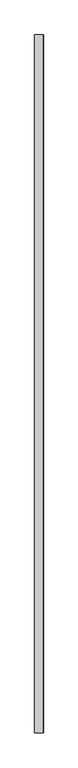
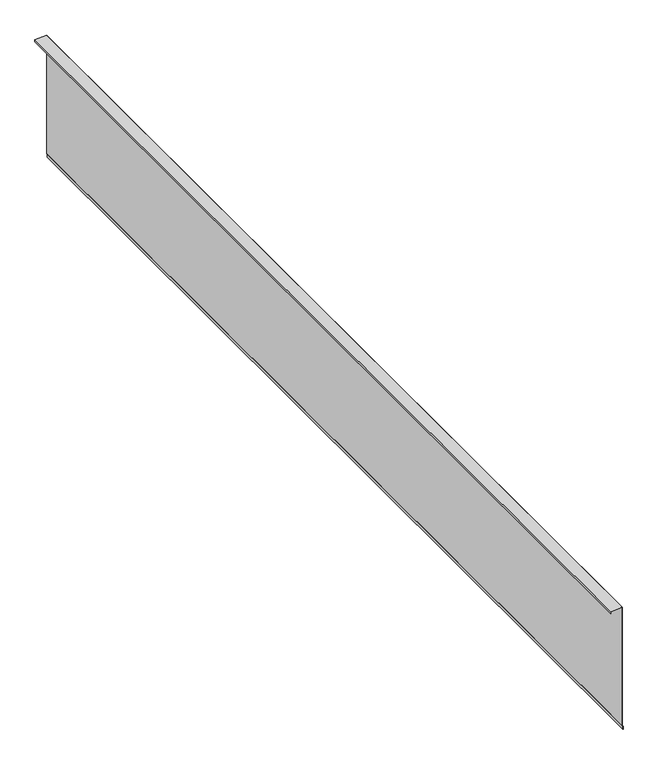
"""IFC4 building model written with IfcOpenShell, lengths in millimetres: proxy geometry, Generic Models 7:Generic Models 1:5:Generic Models 1:5 : Generic Models 7:Generic Models 1:337419:28 : Generic Models 7:Generic Models 1:5:Generic Models 1:5 : Generic Models 7:Generic Models 1:337419:311462."""

from ifc_helpers import new_model, si_unit, frame, origin, place, context, project, spatial, polyline, outline, extrude, source, transform, mapped, element, save


def generic_models_722ccff6(model_context):
    return source(origin(), model_context, "Body", "SweptSolid", [
        extrude(outline(polyline([(0.0, 0.0), (20.1758441, -1e-07), (64.4371907, 30.9921285), (65.3477433, 29.6917246), (20.6763809, -1.5875), (0.5005368, -1.5875), (-1952.5403074, -1369.1214216), (-2070.4890131, -1180.3640352), (-2034.5717889, -1155.2145241), (-2033.6612363, -1156.514928), (-2068.3444233, -1180.8003569), (-1952.0805203, -1366.8614955), (0.0, 0.0)])), frame((579321.2054739, -579019.7413841, 3795.8885169), z_axis=(1.0439982212062661e-11, 1.0, 0.0), x_axis=(0.5735764363524188, -5.988127792777543e-12, -0.8191520442880308)), (0.0, 0.0, 1.0), 18974.5924408),
    ])


if __name__ == "__main__":
    model = new_model("IFC4")
    model_context = context("Model", 3, world=origin())
    ifc_project = project(units=[si_unit("LENGTHUNIT", "METRE", prefix="MILLI")], contexts=[model_context])
    site = spatial("IfcSite", under=ifc_project)
    building = spatial("IfcBuilding", under=site)
    placement = place(None, origin())
    generic_models_shape = generic_models_722ccff6(model_context)
    element("IfcBuildingElementProxy", 1, Name="Generic Models 7:Generic Models 1:5:Generic Models 1:5 : Generic Models 7:Generic Models 1:337419:28 : Generic Models 7:Generic Models 1:5:Generic Models 1:5 : Generic Models 7:Generic Models 1:337419:311462", ObjectType="Generic Models 7:Generic Models 1:5:Generic Models 1:5 : Generic Models 7:Generic Models 1:337419:28 : Generic Models 7:Generic Models 1:5:Generic Models 1:5 : Generic Models 7:Generic Models 1:337419:311462", at=placement, inside=building, context=model_context, shape_type="MappedRepresentation", body=[
        mapped(generic_models_shape, transform((0.0, 0.0, 0.0), x_axis=(1.0, 0.0, 0.0), y_axis=(0.0, 1.0, 0.0), z_axis=(0.0, 0.0, 1.0))),
    ])
    save(model, "model.ifc")

# Revit data of these elements
# Type "Generic Models 7:Generic Models 1:5:Generic Models 1:5 : Generic Models 7:Generic Models 1:337419:28 : Generic Models 7:Generic Models 1:5:Generic Models 1:5 : Generic Models 7:Generic Models 1:337419:311462"
#   NameOverride = "Generic Models 7:Generic Models 1:5:Generic Models 1:5 : Generic Models 7:Generic Models 1:337419:311462"
#   ObjectTypeOverride = "Generic Models 1:5 : Generic Models 7:Generic Models 1:337419"
#   Reference = "Generic Models 1"
#   Tag = "311462"
# Element 1 (IfcBuildingElementProxy, "Generic Models 7:Generic Models 1:5:Generic Models 1:5 : Generic Models 7:Generic Models 1:337419:28 : Generic Models 7:Generic Models 1:5:Generic Models 1:5 : Generic Models 7:Generic Models 1:337419:311462")
#   Materials on its faces: "UV STABLE WATER RESISTANT VAPOR PERMEABLE AIR BARRIER"
# Materials
#   "UV STABLE WATER RESISTANT VAPOR PERMEABLE AIR BARRIER": class "Generic", colour RGB 51 162 45, transparency 0, Description = "Polyethylene film membrane", Cost = 0
